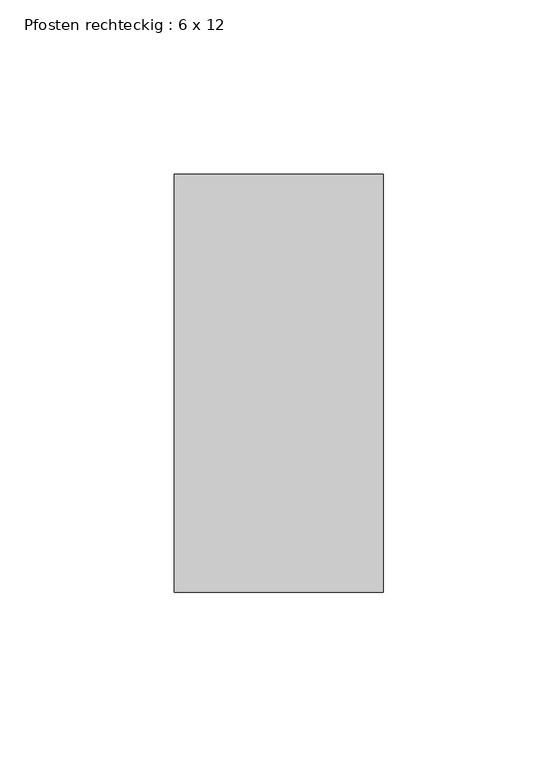
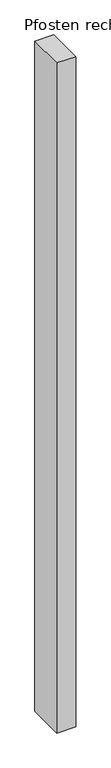
"""IFC4 building model written with IfcOpenShell, lengths in millimetres: member geometry, Pfosten rechteckig : 6 x 12."""

from ifc_helpers import new_model, si_unit, frame, origin, place, context, project, spatial, polyline, outline, extrude, source, transform, mapped, element, save


def pfosten_rechteckig_6_x_12_b6f87324(model_context):
    return source(origin(), model_context, "Body", "SweptSolid", [
        extrude(outline(polyline([(0.0, 60.0), (0.0, -60.0), (-60.0, -60.0), (-60.0, 60.0), (0.0, 60.0)])), frame((0.0, 0.0, -2250.0), z_axis=(0.0, 0.0, 1.0), x_axis=(1.0, 0.0, 0.0)), (0.0, 0.0, 1.0), 2250.0),
    ])


if __name__ == "__main__":
    model = new_model("IFC4")
    model_context = context("Model", 3, world=origin())
    ifc_project = project(units=[si_unit("LENGTHUNIT", "METRE", prefix="MILLI")], contexts=[model_context])
    site = spatial("IfcSite", under=ifc_project)
    building = spatial("IfcBuilding", under=site)
    placement = place(None, origin())
    pfosten_rechteckig_6_x_12_shape = pfosten_rechteckig_6_x_12_b6f87324(model_context)
    element("IfcMember", 1, ObjectType="Pfosten rechteckig : 6 x 12", at=placement, inside=building, context=model_context, shape_type="MappedRepresentation", body=[
        mapped(pfosten_rechteckig_6_x_12_shape, transform((0.0, 0.0, 0.0), x_axis=(1.0, 0.0, 0.0), y_axis=(0.0, 1.0, 0.0), z_axis=(0.0, 0.0, 1.0))),
    ])
    save(model, "model.ifc")

# Revit data of these elements
# Type "Pfosten rechteckig : 6 x 12"
#   built-in parameter 1007304 = 0.393701 (stored number, unit not read)
#   built-in parameter 1007301 = 0.0984252 (stored number, unit not read)
#   built-in parameter 1007300 = 0.0984252 (stored number, unit not read)
# Element 1 (IfcMember, "Pfosten rechteckig : 6 x 12")
#   Materials on its faces: "Metall - verzinkt"
# Materials
#   "Metall - verzinkt": class "Allgemeines", colour RGB 200 200 200, transparency 0, Cost = 0
